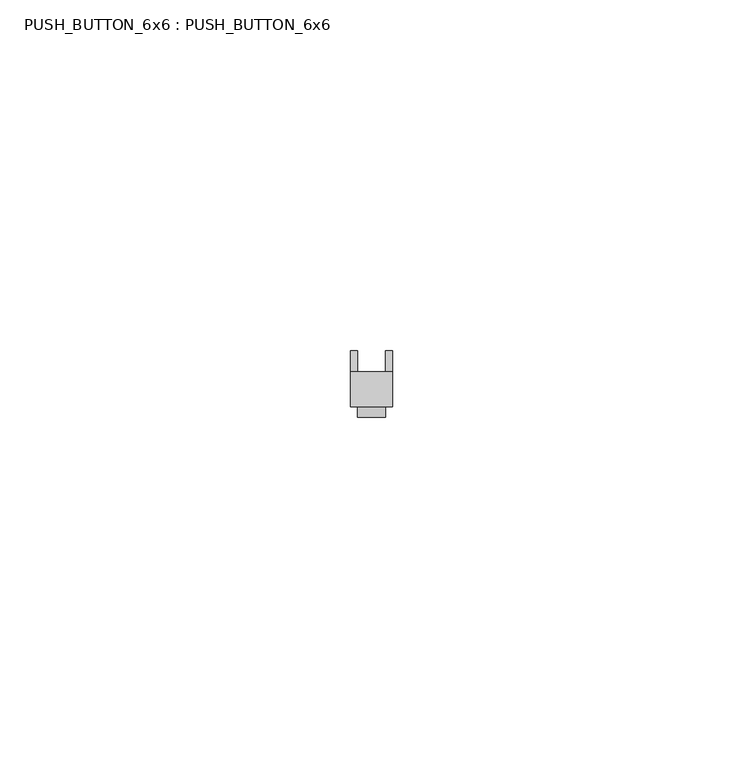
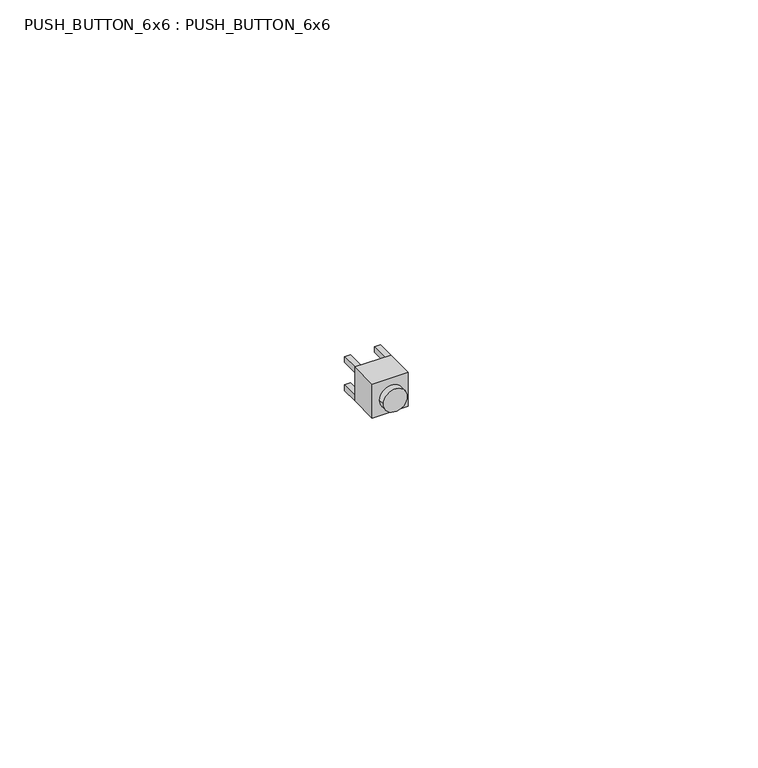
"""IFC4 building model written with IfcOpenShell, lengths in millimetres: furniture geometry, PUSH_BUTTON_6x6 : PUSH_BUTTON_6x6."""

import ifcopenshell
import ifcopenshell.guid

model = None  # the IFC model being written
_history = None  # IfcOwnerHistory: only IFC2X3 demands one
_inside = {}  # id of a spatial element -> (the spatial element, [elements in it])
_under = {}  # id of a project, library or spatial element -> (it, [spatial elements below it])
_declared = {}  # id of a project -> (the project, [libraries it declares])
_typed = {}  # id of a type object -> (the type object, [elements of that type])
_made_of = {}  # id of a material, layer set ... -> (it, [elements and type objects made of it])


def new_model(schema):
    """Start an empty IFC model of exactly this schema.

    Asked for "IFC4X3", IfcOpenShell would pick the latest addendum, in which some entities
    have other attributes; the version numbers below select the first issue.
    IFC2X3 requires an IfcOwnerHistory on every rooted entity: one is made here for all.
    """
    global model, _history
    if schema == "IFC4X3":
        model = ifcopenshell.file(schema_version=(4, 3, 0, 0))
    else:
        model = ifcopenshell.file(schema=schema)
    _inside.clear()
    _under.clear()
    _declared.clear()
    _typed.clear()
    _made_of.clear()
    _history = None
    if model.schema == "IFC2X3":
        org = make("IfcOrganization", Name="unknown")
        user = make(
            "IfcPersonAndOrganization",
            ThePerson=make("IfcPerson", FamilyName="unknown"),
            TheOrganization=org,
        )
        app = make(
            "IfcApplication",
            ApplicationDeveloper=org,
            Version="unknown",
            ApplicationFullName="unknown",
            ApplicationIdentifier="unknown",
        )
        _history = make(
            "IfcOwnerHistory",
            OwningUser=user,
            OwningApplication=app,
            ChangeAction="ADDED",
            CreationDate=0,
        )
    return model


def make(cls, **values):
    """One entity of the class cls with the attributes given. An attribute that is None is left unset."""
    return model.create_entity(
        cls, **{name: value for name, value in values.items() if value is not None}
    )


def rooted(cls, **values):
    """An entity with a GlobalId (a new one), such as an element, a storey or a relation."""
    return make(cls, GlobalId=ifcopenshell.guid.new(), OwnerHistory=_history, **values)


def si_unit(unit_type, name, prefix=None):
    """IfcSIUnit, for example si_unit("LENGTHUNIT", "METRE", prefix="MILLI")."""
    return make("IfcSIUnit", UnitType=unit_type, Prefix=prefix, Name=name)


def assignment(units):
    """IfcUnitAssignment: the units of a project."""
    return None if units is None else make("IfcUnitAssignment", Units=units)


def point(xyz):
    """IfcCartesianPoint."""
    return None if xyz is None else make("IfcCartesianPoint", Coordinates=xyz)


def direction(xyz):
    """IfcDirection."""
    return None if xyz is None else make("IfcDirection", DirectionRatios=xyz)


def frame(location, z_axis=None, x_axis=None):
    """IfcAxis2Placement3D, a coordinate frame: its origin and axes. An axis left out is left unset."""
    return make(
        "IfcAxis2Placement3D",
        Location=point(location),
        Axis=direction(z_axis),
        RefDirection=direction(x_axis),
    )


def frame_2d(location, x_axis=None):
    """IfcAxis2Placement2D, a coordinate frame in the plane: its origin and x axis."""
    return make(
        "IfcAxis2Placement2D", Location=point(location), RefDirection=direction(x_axis)
    )


def origin():
    """The frame at (0, 0, 0) with its axes left unset."""
    return frame((0.0, 0.0, 0.0))


def origin_with_axes():
    """The frame at (0, 0, 0) with the z axis (0, 0, 1) and the x axis (1, 0, 0) written out."""
    return frame((0.0, 0.0, 0.0), z_axis=(0.0, 0.0, 1.0), x_axis=(1.0, 0.0, 0.0))


def place(relative_to, where):
    """IfcLocalPlacement: puts the frame where relative to a parent placement (None: the world)."""
    return make(
        "IfcLocalPlacement", PlacementRelTo=relative_to, RelativePlacement=where
    )


def context(
    kind, dimensions, precision=None, world=None, true_north=None, identifier=None
):
    """IfcGeometricRepresentationContext, for example the 3D "Model" context."""
    return make(
        "IfcGeometricRepresentationContext",
        ContextIdentifier=identifier,
        ContextType=kind,
        CoordinateSpaceDimension=dimensions,
        Precision=precision,
        WorldCoordinateSystem=world,
        TrueNorth=true_north,
    )


def project(units=None, contexts=None):
    """IfcProject with its units and contexts."""
    return rooted(
        "IfcProject",
        Name="project",
        RepresentationContexts=contexts,
        UnitsInContext=assignment(units),
    )


def spatial(cls, under=None, at=None, **own):
    """A site, building, storey or space (cls), placed at a placement, below another one or the project."""
    s = rooted(cls, ObjectPlacement=at, **own)
    if under is not None:
        _under.setdefault(under.id(), (under, []))[1].append(s)
    return s


def polyline(points):
    """IfcPolyline through the points."""
    return make("IfcPolyline", Points=[point(p) for p in points])


def circle_curve(where, radius):
    """IfcCircle in the frame where."""
    return make("IfcCircle", Position=where, Radius=radius)


def trimmed(basis, trim1, trim2, sense, master):
    """IfcTrimmedCurve: the piece of a basis curve between two trims."""
    return make(
        "IfcTrimmedCurve",
        BasisCurve=basis,
        Trim1=trim1,
        Trim2=trim2,
        SenseAgreement=sense,
        MasterRepresentation=master,
    )


def segment(curve, same_sense, transition):
    """IfcCompositeCurveSegment."""
    return make(
        "IfcCompositeCurveSegment",
        Transition=transition,
        SameSense=same_sense,
        ParentCurve=curve,
    )


def composite_curve(segments, self_intersect=None):
    """IfcCompositeCurve: segments joined end to end."""
    return make("IfcCompositeCurve", Segments=segments, SelfIntersect=self_intersect)


def outline(outer, holes=None, kind="AREA"):
    """IfcArbitraryClosedProfileDef: a profile drawn as a closed curve; with holes, ...WithVoids."""
    if holes is None:
        return make("IfcArbitraryClosedProfileDef", ProfileType=kind, OuterCurve=outer)
    return make(
        "IfcArbitraryProfileDefWithVoids",
        ProfileType=kind,
        OuterCurve=outer,
        InnerCurves=holes,
    )


def extrude(swept, where, along, depth):
    """IfcExtrudedAreaSolid: the profile swept, set in the frame where, extruded along a direction by depth."""
    return make(
        "IfcExtrudedAreaSolid",
        SweptArea=swept,
        Position=where,
        ExtrudedDirection=direction(along),
        Depth=depth,
    )


def shape(context_of_items, identifier, shape_type, items):
    """IfcShapeRepresentation: the items that make up one representation, for example the "Body"."""
    return make(
        "IfcShapeRepresentation",
        ContextOfItems=context_of_items,
        RepresentationIdentifier=identifier,
        RepresentationType=shape_type,
        Items=items,
    )


def source(mapping_origin, context_of_items, identifier, shape_type, items):
    """IfcRepresentationMap: a shape defined once, which mapped items show again and again."""
    return make(
        "IfcRepresentationMap",
        MappingOrigin=mapping_origin,
        MappedRepresentation=shape(context_of_items, identifier, shape_type, items),
    )


def transform(
    local_origin,
    x_axis=None,
    y_axis=None,
    z_axis=None,
    scale=None,
    scale2=None,
    scale3=None,
    uniform=True,
):
    """IfcCartesianTransformationOperator3D, or its non-uniform kind. x_axis, y_axis, z_axis: its Axis1, 2, 3."""
    if uniform:
        return make(
            "IfcCartesianTransformationOperator3D",
            Axis1=direction(x_axis),
            Axis2=direction(y_axis),
            LocalOrigin=point(local_origin),
            Scale=scale,
            Axis3=direction(z_axis),
        )
    return make(
        "IfcCartesianTransformationOperator3DnonUniform",
        Axis1=direction(x_axis),
        Axis2=direction(y_axis),
        LocalOrigin=point(local_origin),
        Scale=scale,
        Axis3=direction(z_axis),
        Scale2=scale2,
        Scale3=scale3,
    )


def mapped(mapping_source, mapping_target):
    """IfcMappedItem: shows the shape of a source again, moved by a transform."""
    return make(
        "IfcMappedItem", MappingSource=mapping_source, MappingTarget=mapping_target
    )


def made_of(thing, what):
    """Note that an element or type object is made of a material, layer set ...; save() writes the relation."""
    if what is not None:
        _made_of.setdefault(what.id(), (what, []))[1].append(thing)
    return thing


def element(
    cls,
    number,
    at=None,
    inside=None,
    cuts=None,
    type_object=None,
    material=None,
    context=None,
    identifier="Body",
    shape_type=None,
    held_by="IfcProductDefinitionShape",
    body=None,
    shapes=None,
    **own,
):
    """One element of the class cls, such as IfcWall. Its Tag is "e" and its number.

    at: its placement. inside: the storey or other place that contains it. cuts: it is an
    opening in that element (IfcRelVoidsElement). A single representation is given by context,
    identifier, shape_type and body (its items); several are given by shapes. held_by: the class
    of the entity that holds the representations. save() writes the other relations.
    """
    e = rooted(cls, Tag="e%d" % number, ObjectPlacement=at, **own)
    if body is not None:
        shapes = [shape(context, identifier, shape_type, body)]
    if shapes is not None:
        e.Representation = make(held_by, Representations=shapes)
    if inside is not None:
        _inside.setdefault(inside.id(), (inside, []))[1].append(e)
    if cuts is not None:
        rooted(
            "IfcRelVoidsElement", RelatingBuildingElement=cuts, RelatedOpeningElement=e
        )
    if type_object is not None:
        _typed.setdefault(type_object.id(), (type_object, []))[1].append(e)
    return made_of(e, material)


def aggregate(whole, parts):
    """IfcRelAggregates: a whole, such as a stair, and the parts it consists of."""
    return rooted("IfcRelAggregates", RelatingObject=whole, RelatedObjects=parts)


def save(model, path):
    """Write the relations noted so far, then the file.

    IfcRelAggregates (storeys below a building ...), IfcRelContainedInSpatialStructure (elements
    in a storey), IfcRelDefinesByType, IfcRelAssociatesMaterial and IfcRelDeclares: one each for
    every whole, place, type object, material and project.
    """
    for whole, parts in _under.values():
        aggregate(whole, parts)
    for where, things in _inside.values():
        rooted(
            "IfcRelContainedInSpatialStructure",
            RelatedElements=things,
            RelatingStructure=where,
        )
    for kind, things in _typed.values():
        rooted("IfcRelDefinesByType", RelatedObjects=things, RelatingType=kind)
    for what, things in _made_of.values():
        rooted("IfcRelAssociatesMaterial", RelatedObjects=things, RelatingMaterial=what)
    for by, libraries in _declared.values():
        rooted("IfcRelDeclares", RelatingContext=by, RelatedDefinitions=libraries)
    model.write(path)


def push_button_6x6_push_button_6x6_b47c84f7(model_context):
    return source(origin(), model_context, "Body", "SweptSolid", [
        extrude(outline(polyline([(-3.0, 0.0), (-3.0, 5.0), (3.0, 5.0), (3.0, 0.0), (-3.0, 0.0)])), origin_with_axes(), (0.0, 0.0, 1.0), 6.0),
        extrude(outline(composite_curve([segment(trimmed(circle_curve(frame_2d((3.0, 0.0)), 2.0), [point((3.0, -2.0))], [point((3.0, 2.0))], False, "CARTESIAN"), True, "CONTINUOUS"), segment(trimmed(circle_curve(frame_2d((3.0, 0.0)), 2.0), [point((3.0, 2.0))], [point((3.0, -2.0))], False, "CARTESIAN"), True, "CONTINUOUS")], self_intersect=False)), frame((0.0, -1.5, 0.0), z_axis=(0.0, 1.0, 0.0), x_axis=(0.0, 0.0, 1.0)), (0.0, 0.0, 1.0), 1.5),
        extrude(outline(polyline([(3.0, 5.0), (2.0, 5.0), (2.0, 8.0), (3.0, 8.0), (3.0, 5.0)])), frame((0.0, 0.0, 5.0), z_axis=(0.0, 0.0, 1.0), x_axis=(1.0, 0.0, 0.0)), (0.0, 0.0, 1.0), 1.0),
        extrude(outline(polyline([(-2.0, 5.0), (-3.0, 5.0), (-3.0, 8.0), (-2.0, 8.0), (-2.0, 5.0)])), frame((0.0, 0.0, 5.0), z_axis=(0.0, 0.0, 1.0), x_axis=(1.0, 0.0, 0.0)), (0.0, 0.0, 1.0), 1.0),
        extrude(outline(polyline([(3.0, 5.0), (2.0, 5.0), (2.0, 8.0), (3.0, 8.0), (3.0, 5.0)])), origin_with_axes(), (0.0, 0.0, 1.0), 1.0),
        extrude(outline(polyline([(-2.0, 5.0), (-3.0, 5.0), (-3.0, 8.0), (-2.0, 8.0), (-2.0, 5.0)])), origin_with_axes(), (0.0, 0.0, 1.0), 1.0),
    ])


if __name__ == "__main__":
    model = new_model("IFC4")
    model_context = context("Model", 3, world=origin())
    ifc_project = project(units=[si_unit("LENGTHUNIT", "METRE", prefix="MILLI")], contexts=[model_context])
    site = spatial("IfcSite", under=ifc_project)
    building = spatial("IfcBuilding", under=site)
    placement = place(None, origin())
    push_button_6x6_push_button_6x6_shape = push_button_6x6_push_button_6x6_b47c84f7(model_context)
    element("IfcFurniture", 1, ObjectType="PUSH_BUTTON_6x6 : PUSH_BUTTON_6x6", at=placement, inside=building, context=model_context, shape_type="MappedRepresentation", body=[
        mapped(push_button_6x6_push_button_6x6_shape, transform((0.0, 0.0, 0.0), x_axis=(1.0, 0.0, 0.0), y_axis=(0.0, 1.0, 0.0), z_axis=(0.0, 0.0, 1.0))),
    ])
    save(model, "model.ifc")

# Revit data of these elements
# Type "PUSH_BUTTON_6x6 : PUSH_BUTTON_6x6"
#   Default Elevation = 0
# Element 1 (IfcFurniture, "PUSH_BUTTON_6x6 : PUSH_BUTTON_6x6")
#   Materials on its faces: ".BOTAO"
# Materials
#   ".BOTAO": class "Vidro", colour RGB 0 255 255, transparency 0.75, Cost = 0
